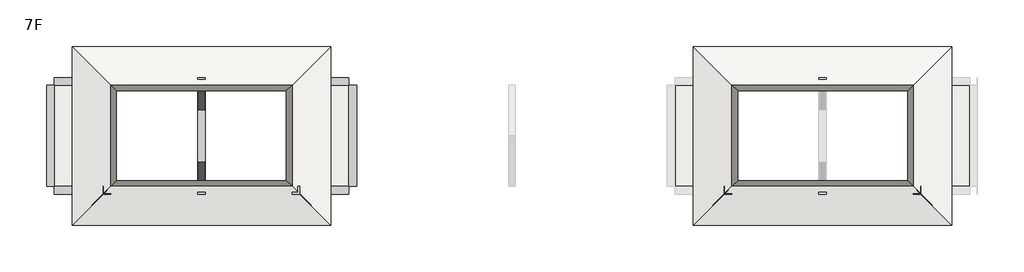
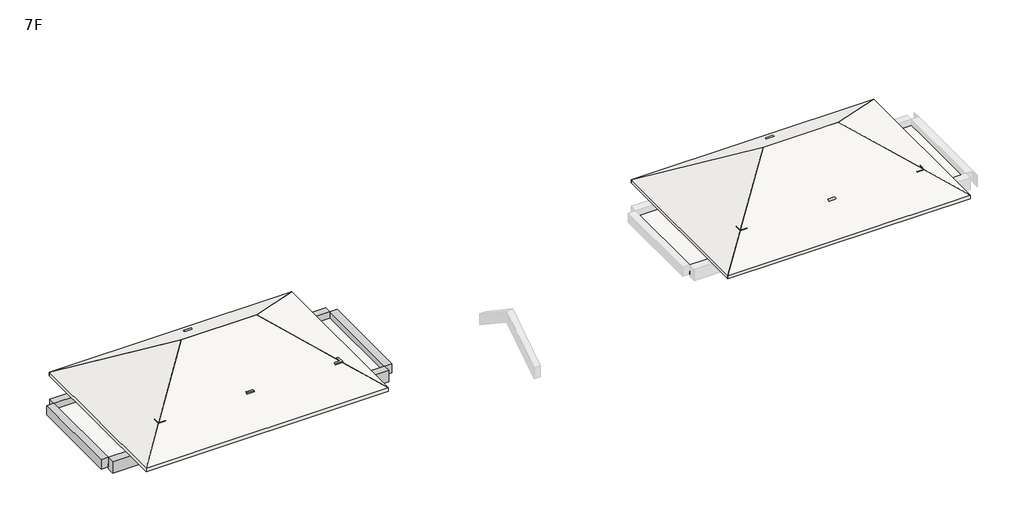
# One storey, part 1 of 2: 15 beams, 9 slabs, 5 columns.
"""IFC4 building model written with IfcOpenShell, lengths in millimetres."""

from ifc_helpers import new_model, si_unit, frame, origin, place, context, project, spatial, polyline, outline, extrude, faceted_brep, element, save

model = new_model("IFC4")

# Units and contexts
model_context = context("Model", 3, world=origin())
ifc_project = project(units=[si_unit("LENGTHUNIT", "METRE", prefix="MILLI")], contexts=[model_context])

# Site, building, storey
site = spatial("IfcSite", under=ifc_project)
building = spatial("IfcBuilding", under=site)
storey = spatial("IfcBuildingStorey", under=building, Name="7F", Elevation=20530.0)

# Beams
placement = place(None, origin())
element("IfcBeam", 1, ObjectType="M_Concrete-Rectangular Beam : 250x400", at=placement, inside=storey, context=model_context, shape_type="SweptSolid", body=[
    extrude(outline(polyline([(9399.8746382, 8450.0000002), (9649.8746382, 8450.0000002), (9649.8746382, 4549.9999996), (9399.8746382, 4549.9999996), (9399.8746382, 8450.0000002)])), frame((0.0, 0.0, 20130.0), z_axis=(0.0, 0.0, 1.0), x_axis=(1.0, 0.0, 0.0)), (0.0, 0.0, 1.0), 400.0),
])
element("IfcBeam", 2, ObjectType="M_Concrete-Rectangular Beam : 250x400", at=placement, inside=storey, context=model_context, shape_type="SweptSolid", body=[
    extrude(outline(polyline([(2050.1253632, 8450.0000002), (2300.1253632, 8450.0000002), (2300.1253632, 4549.9999996), (2050.1253632, 4549.9999996), (2050.1253632, 8450.0000002)])), frame((0.0, 0.0, 20130.0), z_axis=(0.0, 0.0, 1.0), x_axis=(1.0, 0.0, 0.0)), (0.0, 0.0, 1.0), 400.0),
])
element("IfcBeam", 3, ObjectType="M_Concrete-Rectangular Beam : 250x400", at=placement, inside=storey, context=model_context, shape_type="Brep", body=[
    faceted_brep([(5725.0000684, 6499.7375861, 22885.8347272), (5975.0000684, 6499.7375861, 22885.8347272), (5975.0000684, 8449.9999997, 21585.6270796), (5725.0000684, 8449.9999997, 21585.6270796), (5725.0000684, 6277.8536437, 22553.0171854), (5725.0000684, 8449.9999997, 21104.8831887), (5725.0000684, 6499.7375861, 22405.0908362), (5975.0000684, 6277.8536437, 22553.0171854), (5975.0000684, 8449.9999997, 21104.8831887), (5975.0000684, 6499.7375861, 22405.0908362)], [[[0, 1, 2, 3]], [[4, 0, 3, 5, 6]], [[7, 4, 6, 5, 8, 9]], [[1, 7, 9, 8, 2]], [[1, 0, 4, 7]], [[3, 2, 8, 5]]]),
])
element("IfcBeam", 4, ObjectType="M_Concrete-Rectangular Beam : 250x400", at=placement, inside=storey, context=model_context, shape_type="SweptSolid", body=[
    extrude(outline(polyline([(6277.8536437, 22553.0171854), (6499.7375861, 22405.0908362), (4549.9999992, 21105.2330819), (4549.9999992, 21585.9769728), (6499.7375861, 22885.8347272), (6277.8536437, 22553.0171854)])), frame((5725.0000684, 0.0, 0.0), z_axis=(1.0, 0.0, 0.0), x_axis=(0.0, 1.0, 0.0)), (0.0, 0.0, 1.0), 250.0),
])
element("IfcBeam", 5, ObjectType="M_Concrete-Rectangular Beam : 250x400", at=placement, inside=storey, context=model_context, shape_type="Brep", body=[
    faceted_brep([(9629.9825629, 4549.9999992, 21480.0), (9629.9825629, 8724.9999993, 21480.0), (9625.1196449, 8724.9999993, 21480.0), (9508.5592132, 8608.4366337, 21480.0), (9379.9825629, 8608.4366337, 21480.0), (9379.9825629, 8474.9999993, 21480.0), (9379.9825629, 4549.9999992, 21480.0), (9379.9825629, 4549.9999992, 21080.0), (9379.9825629, 8655.7227157, 21448.4751524), (9379.9825629, 8474.9999993, 21448.4751524), (9379.9825629, 8449.9999997, 21448.4751524), (9379.9825629, 8449.9999997, 21080.0), (9629.9825629, 4549.9999992, 21080.0), (9629.9825629, 8449.9999997, 21080.0), (9629.9825629, 8449.9999997, 21448.4751524), (9629.9825629, 8724.9999993, 21448.4751524), (9625.1196449, 8724.9999993, 21448.4751524), (9555.844105, 8655.7227157, 21448.4751524)], [[[0, 1, 2, 3, 4, 5, 6]], [[7, 6, 5, 4, 8, 9, 10, 11]], [[12, 7, 11, 13]], [[1, 0, 12, 13, 14, 15]], [[1, 15, 16, 2]], [[0, 6, 7, 12]], [[10, 14, 13, 11]], [[14, 10, 9, 8, 17, 16, 15]], [[3, 17, 8, 4]], [[17, 3, 2, 16]]]),
])
element("IfcBeam", 6, ObjectType="M_Concrete-Rectangular Beam : 250x400", at=placement, inside=storey, context=model_context, shape_type="SweptSolid", body=[
    extrude(outline(polyline([(21080.0, 2075.0175574), (21080.0, 2325.0175574), (21480.0, 2325.0175574), (21480.0, 2191.5713212), (21402.3014348, 2075.0175574), (21080.0, 2075.0175574)])), frame((0.0, 4549.9999992, 0.0), z_axis=(0.0, 1.0, 0.0), x_axis=(0.0, 0.0, 1.0)), (0.0, 0.0, 1.0), 3887.3000005),
])
element("IfcBeam", 7, ObjectType="M_Concrete-Rectangular Beam : 250x400", at=placement, inside=storey, context=model_context, shape_type="Brep", body=[
    faceted_brep([(5999.9855405, 8474.9999993, 21480.0), (9379.9825629, 8474.9999993, 21480.0), (9379.9825629, 8608.4366337, 21480.0), (5999.9855405, 8608.4366337, 21480.0), (9379.9825629, 8474.9999993, 21448.4751524), (5999.9855405, 8474.9999993, 21080.0), (9349.8746382, 8474.9999993, 21080.0), (9349.8746382, 8474.9999993, 21448.4751524), (9349.8746382, 8724.9999993, 21080.0), (5999.9855405, 8724.9999993, 21080.0), (5999.9855405, 8724.9999993, 21402.2891349), (9349.8746382, 8724.9999993, 21402.2891349), (9379.9825629, 8655.7227157, 21448.4751524), (9349.8746382, 8655.7227157, 21448.4751524)], [[[0, 1, 2, 3]], [[4, 1, 0, 5, 6, 7]], [[8, 6, 5, 9]], [[8, 9, 10, 11]], [[1, 4, 12, 2]], [[7, 6, 8, 11, 13]], [[4, 7, 13, 12]], [[5, 0, 3, 10, 9]], [[3, 2, 12, 13, 11, 10]]]),
    faceted_brep([(2075.0175574, 8474.9999993, 21448.4751524), (2075.0175574, 8474.9999993, 21480.0), (2075.0175574, 8724.7509238, 21480.0), (2075.0175574, 8724.7509238, 21448.4751524), (2350.1253632, 8474.9999993, 21080.0), (2350.1253632, 8474.9999993, 21448.4751524), (2350.1253632, 8655.7227157, 21448.4751524), (2350.1253632, 8724.9999993, 21402.2891349), (2350.1253632, 8724.9999993, 21080.0), (2144.0475031, 8655.7227157, 21448.4751524), (5699.9855405, 8474.9999993, 21480.0), (5699.9855405, 8474.9999993, 21080.0), (5699.9855405, 8724.9999993, 21080.0), (5699.9855405, 8724.9999993, 21402.2891349), (5699.9855405, 8608.4366337, 21480.0), (2191.3347752, 8608.4366337, 21480.0)], [[[0, 1, 2, 3]], [[4, 5, 6, 7, 8]], [[5, 0, 3, 9, 6]], [[10, 11, 12, 13, 14]], [[1, 10, 14, 15, 2]], [[1, 0, 5, 4, 11, 10]], [[4, 8, 12, 11]], [[12, 8, 7, 13]], [[15, 9, 3, 2]], [[9, 15, 14, 13, 7, 6]]]),
])
element("IfcBeam", 8, ObjectType="M_Concrete-Rectangular Beam : 250x400", at=placement, inside=storey, context=model_context, shape_type="SweptSolid", body=[
    extrude(outline(polyline([(4524.9999902, 21080.0), (4274.9999902, 21080.0), (4274.9999902, 21402.6390255), (4391.0385331, 21480.0), (4524.9999902, 21480.0), (4524.9999902, 21080.0)])), frame((5999.9855405, 0.0, 0.0), z_axis=(1.0, 0.0, 0.0), x_axis=(0.0, 1.0, 0.0)), (0.0, 0.0, 1.0), 3349.8890977),
    extrude(outline(polyline([(4524.9999902, 21480.0), (4524.9999902, 21080.0), (4274.9999902, 21080.0), (4274.9999902, 21402.6390255), (4391.0385331, 21480.0), (4524.9999902, 21480.0)])), frame((2350.0175574, 0.0, 0.0), z_axis=(1.0, 0.0, 0.0), x_axis=(0.0, 1.0, 0.0)), (0.0, 0.0, 1.0), 3349.9679831),
])
element("IfcBeam", 9, ObjectType="M_Concrete-Rectangular Beam : 300x400", at=placement, inside=storey, context=model_context, shape_type="SweptSolid", body=[
    extrude(outline(polyline([(165.0, 4549.9999996), (-135.0, 4549.9999996), (-135.0, 8450.0000002), (165.0, 8450.0000002), (165.0, 4549.9999996)])), frame((0.0, 0.0, 20130.0), z_axis=(0.0, 0.0, 1.0), x_axis=(1.0, 0.0, 0.0)), (0.0, 0.0, 1.0), 400.0),
])
element("IfcBeam", 10, ObjectType="M_Concrete-Rectangular Beam : 300x400", at=placement, inside=storey, context=model_context, shape_type="SweptSolid", body=[
    extrude(outline(polyline([(11550.0174941, 8450.0000002), (11850.0174941, 8450.0000002), (11850.0174941, 4549.9999996), (11550.0174941, 4549.9999996), (11550.0174941, 8450.0000002)])), frame((0.0, 0.0, 20130.0), z_axis=(0.0, 0.0, 1.0), x_axis=(1.0, 0.0, 0.0)), (0.0, 0.0, 1.0), 400.0),
])
element("IfcBeam", 11, ObjectType="M_Concrete-Rectangular Beam : 300x400", at=placement, inside=storey, context=model_context, shape_type="Brep", body=[
    faceted_brep([(6000.0, 8450.0000002, 20530.0), (5700.0, 8450.0000002, 20530.0), (5700.0, 4549.9999996, 20530.0), (6000.0, 4550.0000005, 20530.0), (6000.0, 4550.0000005, 20130.0), (6000.0, 8450.0000002, 20130.0), (5700.0, 8450.0000002, 20130.0), (5700.0, 4549.9999996, 20130.0)], [[[0, 1, 2, 3]], [[3, 4, 5, 0]], [[6, 5, 4, 7]], [[1, 6, 7, 2]], [[0, 5, 6, 1]], [[2, 7, 4, 3]]]),
])
element("IfcBeam", 12, ObjectType="M_Concrete-Rectangular Beam : 300x500", at=placement, inside=storey, context=model_context, shape_type="Brep", body=[
    faceted_brep([(164.9649925, 8750.0000002, 20530.0), (164.9649925, 8450.0000002, 20530.0), (2050.1253632, 8450.0000002, 20530.0), (2300.1253632, 8450.0000002, 20530.0), (5700.0000012, 8450.0000002, 20530.0), (5700.0000012, 8750.0000002, 20530.0), (164.9649925, 8450.0000002, 20030.0), (5700.0000012, 8450.0000002, 20030.0), (164.9649925, 8750.0000002, 20030.0), (5700.0000012, 8750.0000002, 20030.0)], [[[0, 1, 2, 3, 4, 5]], [[1, 6, 7, 4, 3, 2]], [[6, 8, 9, 7]], [[8, 0, 5, 9]], [[1, 0, 8, 6]], [[5, 4, 7, 9]]]),
])
element("IfcBeam", 13, ObjectType="M_Concrete-Rectangular Beam : 300x500", at=placement, inside=storey, context=model_context, shape_type="Brep", body=[
    faceted_brep([(164.9649925, 4549.9999996, 20530.0), (164.9649925, 4249.9999996, 20530.0), (5700.0000012, 4249.9999996, 20530.0), (5700.0000012, 4549.9999996, 20530.0), (2300.1253632, 4549.9999996, 20530.0), (2050.1253632, 4549.9999996, 20530.0), (164.9649925, 4249.9999996, 20030.0), (5700.0000012, 4249.9999996, 20030.0), (164.9649925, 4549.9999996, 20030.0), (5700.0000012, 4549.9999996, 20030.0)], [[[0, 1, 2, 3, 4, 5]], [[1, 6, 7, 2]], [[6, 8, 9, 7]], [[8, 0, 5, 4, 3, 9]], [[1, 0, 8, 6]], [[3, 2, 7, 9]]]),
])
element("IfcBeam", 14, ObjectType="M_Concrete-Rectangular Beam : 300x500", at=placement, inside=storey, context=model_context, shape_type="Brep", body=[
    faceted_brep([(6000.0000012, 8750.0000002, 20530.0), (6000.0, 8450.0000002, 20530.0), (9399.8746382, 8450.0000002, 20530.0), (9649.8746382, 8450.0000002, 20530.0), (11550.000003, 8450.0000002, 20530.0), (11550.000003, 8750.0000002, 20530.0), (6000.0000012, 8450.0000002, 20030.0), (11550.000003, 8450.0000002, 20030.0), (6000.0000012, 8750.0000002, 20030.0), (11550.000003, 8750.0000002, 20030.0)], [[[0, 1, 2, 3, 4, 5]], [[1, 6, 7, 4, 3, 2]], [[6, 8, 9, 7]], [[8, 0, 5, 9]], [[8, 6, 1, 0]], [[5, 4, 7, 9]]]),
])
element("IfcBeam", 15, ObjectType="M_Concrete-Rectangular Beam : 300x500", at=placement, inside=storey, context=model_context, shape_type="Brep", body=[
    faceted_brep([(6000.0, 4549.9999996, 20530.0), (6000.0000012, 4249.9999996, 20530.0), (11550.000003, 4249.9999996, 20530.0), (11550.000003, 4549.9999996, 20530.0), (9649.8746382, 4549.9999996, 20530.0), (9399.8746382, 4549.9999996, 20530.0), (6000.0000012, 4249.9999996, 20030.0), (11550.000003, 4249.9999996, 20030.0), (6000.0000012, 4549.9999996, 20030.0), (11550.000003, 4549.9999996, 20030.0)], [[[0, 1, 2, 3, 4, 5]], [[1, 6, 7, 2]], [[6, 8, 9, 7]], [[8, 0, 5, 4, 3, 9]], [[8, 6, 1, 0]], [[3, 2, 7, 9]]]),
])

# Columns
element("IfcColumn", 16, ObjectType="M_Concrete-Rectangular-Column : 300x300", at=placement, inside=storey, context=model_context, shape_type="Brep", body=[
    faceted_brep([(5999.9855405, 4549.9999992, 20530.0), (5999.9855405, 4249.9999992, 20530.0), (5699.9855405, 4249.9999992, 20530.0), (5699.9855405, 4549.9999992, 20530.0), (5699.9855405, 4549.9999992, 21585.9769764), (5999.9855405, 4549.9999992, 21585.9769764), (5999.9855405, 4249.9999992, 21385.9719455), (5999.9855405, 4274.9999902, 21402.6390255), (5999.9855405, 4391.0385331, 21480.0), (5699.9855405, 4391.0385331, 21480.0), (5699.9855405, 4274.9999902, 21402.6390255), (5699.9855405, 4249.9999992, 21385.9719455)], [[[0, 1, 2, 3]], [[0, 3, 4, 5]], [[6, 7, 8, 5, 4, 9, 10, 11]], [[1, 0, 5, 8, 7, 6]], [[2, 1, 6, 11]], [[3, 2, 11, 10, 9, 4]]]),
    faceted_brep([(5999.9855405, 4249.9999992, 21585.9769764), (5999.9855405, 4249.9999992, 21530.1951128), (5999.9855405, 4333.6706899, 21585.9769764), (5699.9855405, 4249.9999992, 21585.9769764), (5699.9855405, 4249.9999992, 21530.1951128), (5699.9855405, 4333.6706899, 21585.9769764)], [[[0, 1, 2]], [[0, 3, 4, 1]], [[4, 3, 5]], [[3, 0, 2, 5]], [[2, 1, 4, 5]]]),
])
element("IfcColumn", 17, ObjectType="M_Concrete-Rectangular-Column : 300x300", at=placement, inside=storey, context=model_context, shape_type="Brep", body=[
    faceted_brep([(5999.9855405, 8749.9999997, 20530.0), (5999.9855405, 8449.9999997, 20530.0), (5699.9855405, 8449.9999997, 20530.0), (5699.9855405, 8749.9999997, 20530.0), (5999.9855405, 8449.9999997, 21585.6270796), (5699.9855405, 8449.9999997, 21585.6270796), (5999.9855405, 8608.4366337, 21480.0), (5999.9855405, 8724.9999993, 21402.2891349), (5999.9855405, 8749.9999997, 21385.6220487), (5699.9855405, 8749.9999997, 21385.6220487), (5699.9855405, 8724.9999993, 21402.2891349), (5699.9855405, 8608.4366337, 21480.0)], [[[0, 1, 2, 3]], [[2, 1, 4, 5]], [[4, 6, 7, 8, 9, 10, 11, 5]], [[1, 0, 8, 7, 6, 4]], [[3, 2, 5, 11, 10, 9]], [[0, 3, 9, 8]]]),
    faceted_brep([(5999.9855405, 8749.9999997, 21529.845216), (5999.9855405, 8749.9999997, 21585.6270796), (5999.9855405, 8666.329309, 21585.6270796), (5699.9855405, 8749.9999997, 21585.6270796), (5699.9855405, 8749.9999997, 21529.845216), (5699.9855405, 8666.329309, 21585.6270796)], [[[0, 1, 2]], [[3, 4, 5]], [[3, 1, 0, 4]], [[1, 3, 5, 2]], [[0, 2, 5, 4]]]),
])
element("IfcColumn", 18, ObjectType="M_Concrete-Rectangular-Column : 300x300", at=placement, inside=storey, context=model_context, shape_type="Brep", body=[
    faceted_brep([(9649.8746382, 4549.9999992, 20530.0), (9649.8746382, 4249.9999992, 20530.0), (9349.8746382, 4249.9999992, 20530.0), (9349.8746382, 4549.9999992, 20530.0), (9649.8746382, 4549.9999992, 21585.6973295), (9649.8746382, 4249.9999992, 21585.6973295), (9649.8746382, 4249.9999992, 21529.9272796), (9649.8746382, 4549.9999992, 21529.9272796), (9649.8746382, 4249.9999992, 21385.7074809), (9649.5941992, 4249.9999992, 21385.8944308), (9649.5941992, 4249.9999992, 21530.1142294), (9349.8746382, 4249.9999992, 21585.6973295), (9349.8746382, 4549.7271047, 21585.6973295), (9349.8746382, 4549.9999992, 21585.6973295), (9566.2153171, 4549.9999992, 21585.6973295), (9566.2153171, 4333.3809801, 21585.6973295), (9649.8746382, 4549.9999992, 21385.7074809)], [[[0, 1, 2, 3]], [[4, 5, 6, 7]], [[2, 1, 8, 9, 10, 6, 5, 11]], [[3, 2, 11, 12, 13]], [[4, 7, 14]], [[5, 4, 14, 15, 12, 11]], [[12, 9, 8, 16, 13]], [[10, 15, 14, 7, 6]], [[9, 12, 15, 10]], [[1, 0, 16, 8]], [[0, 3, 13, 16]]]),
])
element("IfcColumn", 19, ObjectType="M_Concrete-Rectangular-Column : 300x300", at=placement, inside=storey, context=model_context, shape_type="Brep", body=[
    faceted_brep([(2350.1253632, 4549.9999992, 20530.0), (2350.1253632, 4249.9999992, 20530.0), (2050.1253632, 4249.9999992, 20530.0), (2050.1253632, 4549.9999992, 20530.0), (2350.1253632, 4549.9999992, 21544.1224713), (2350.1253632, 4249.9999992, 21544.1224713), (2050.1253632, 4249.9999992, 21544.1224713), (2050.1253632, 4249.9999992, 21529.9272796), (2050.4058022, 4249.9999992, 21530.1142294), (2050.4058022, 4249.9999992, 21385.8944308), (2050.1253632, 4249.9999992, 21385.7074809), (2050.1253632, 4549.9999992, 21544.1224713), (2050.1253632, 4549.9999992, 21529.9272796), (2071.4192316, 4549.9999992, 21544.1224713), (2287.7599104, 4549.9999992, 21544.1224713), (2287.7599104, 4487.360082, 21544.1224713), (2071.4192316, 4271.0139574, 21544.1224713), (2050.1253632, 4549.9999992, 21385.7074809)], [[[0, 1, 2, 3]], [[1, 0, 4, 5]], [[2, 1, 5, 6, 7, 8, 9, 10]], [[6, 11, 12, 7]], [[12, 11, 13]], [[5, 4, 14, 15, 16, 13, 11, 6]], [[9, 15, 14, 17, 10]], [[16, 8, 7, 12, 13]], [[15, 9, 8, 16]], [[3, 2, 10, 17]], [[0, 3, 17, 14, 4]]]),
])
element("IfcColumn", 20, ObjectType="M_Concrete-Rectangular-Column : 300x300", at=placement, inside=storey, context=model_context, shape_type="Brep", body=[
    faceted_brep([(2350.1253632, 8749.9999997, 20530.0), (2350.1253632, 8449.9999997, 20530.0), (2050.1253632, 8449.9999997, 20530.0), (2050.1253632, 8749.9999997, 20530.0), (2350.1253632, 8749.9999997, 21385.6220487), (2350.1253632, 8655.7227157, 21448.4751524), (2350.1253632, 8449.9999997, 21448.4751524), (2050.1253632, 8449.9999997, 21448.4751524), (2050.1253632, 8749.6424915, 21448.4751524), (2050.1253632, 8749.6424915, 21385.8603935), (2050.1253632, 8749.9999997, 21385.6220487), (2144.0475031, 8655.7227157, 21448.4751524)], [[[0, 1, 2, 3]], [[1, 0, 4, 5, 6]], [[2, 1, 6, 7]], [[3, 2, 7, 8, 9, 10]], [[0, 3, 10, 4]], [[7, 6, 5, 11, 8]], [[9, 11, 5, 4, 10]], [[11, 9, 8]]]),
])

# Slabs
element("IfcSlab", 21, ObjectType="120", at=placement, inside=storey, context=model_context, shape_type="Brep", body=[
    faceted_brep([(10849.8264643, 9949.7376449, 20585.7768327), (9555.844105, 8655.7227157, 21448.4751524), (9508.5592132, 8608.4366337, 21480.0), (7400.0000782, 6499.8244256, 22885.7768327), (4300.0000585, 6499.8244256, 22885.7768327), (2191.3347752, 8608.4366337, 21480.0), (2144.0475031, 8655.7227157, 21448.4751524), (2050.1253632, 8749.6424915, 21385.8603935), (850.0000025, 9949.7376449, 20585.7768327), (10849.8264643, 9949.7376449, 20730.0), (850.0000025, 9949.7376449, 20730.0), (4300.0000585, 6499.8244256, 23030.0), (7400.0000782, 6499.8244256, 23030.0)], [[[0, 1, 2, 3, 4, 5, 6, 7, 8]], [[9, 10, 11, 12]], [[0, 8, 10, 9]], [[3, 2, 1, 0, 9, 12]], [[4, 3, 12, 11]], [[8, 7, 6, 5, 4, 11, 10]]]),
])
element("IfcSlab", 22, ObjectType="120", at=placement, inside=storey, context=model_context, shape_type="Brep", body=[
    faceted_brep([(10849.8264639, 9949.7376446, 20585.7802013), (10849.8264639, 3049.7375222, 20585.7802013), (9649.5941992, 4249.9999992, 21385.8944308), (9349.8746382, 4549.7271047, 21585.6973295), (7399.913241, 6499.7375863, 22885.605611), (10849.8264639, 9949.7376446, 20730.0), (7399.913241, 6499.7375863, 23029.8254097), (9566.2153171, 4333.3809801, 21585.6973295), (9649.5941992, 4249.9999992, 21530.1142294), (10849.8264639, 3049.7375222, 20730.0)], [[[0, 1, 2, 3, 4]], [[5, 6, 7, 8, 9]], [[1, 0, 5, 9]], [[4, 3, 2, 1, 9, 8, 7, 6]], [[0, 4, 6, 5]]]),
])
element("IfcSlab", 23, ObjectType="120", at=placement, inside=storey, context=model_context, shape_type="Brep", body=[
    faceted_brep([(10849.8264643, 3049.7375219, 20585.7768327), (850.0000025, 3049.7375219, 20585.7768327), (4300.0000585, 6499.6507412, 22885.7768327), (7400.0000782, 6499.6507412, 22885.7768327), (10849.8264643, 3049.7375219, 20730.0), (7400.0000782, 6499.6507412, 23030.0), (4300.0000585, 6499.6507412, 23030.0), (850.0000025, 3049.7375219, 20730.0)], [[[0, 1, 2, 3]], [[4, 5, 6, 7]], [[1, 0, 4, 7]], [[0, 3, 5, 4]], [[3, 2, 6, 5]], [[2, 1, 7, 6]]]),
])
element("IfcSlab", 24, ObjectType="120", at=placement, inside=storey, context=model_context, shape_type="Brep", body=[
    faceted_brep([(850.1735375, 9949.7376446, 20585.7802013), (4300.0867604, 6499.7375863, 22885.605611), (2287.7599104, 4487.360082, 21544.1224713), (2050.4058022, 4249.9999992, 21385.8944308), (850.1735375, 3049.7375222, 20585.7802013), (850.1735375, 9949.7376446, 20730.0), (850.1735375, 3049.7375222, 20730.0), (2050.4058022, 4249.9999992, 21530.1142294), (2071.4192316, 4271.0139574, 21544.1224713), (4300.0867604, 6499.7375863, 23029.8254097)], [[[0, 1, 2, 3, 4]], [[5, 6, 7, 8, 9]], [[0, 4, 6, 5]], [[4, 3, 2, 1, 9, 8, 7, 6]], [[1, 0, 5, 9]]]),
])
element("IfcSlab", 25, ObjectType="120", at=placement, inside=storey, context=model_context, shape_type="Brep", body=[
    faceted_brep([(34849.8264674, 9949.7376449, 20585.7768327), (33649.8746414, 8749.7556157, 21385.7849755), (33555.8441081, 8655.7227157, 21448.4751524), (33508.5592163, 8608.4366337, 21480.0), (31400.0000814, 6499.8244256, 22885.7768327), (28300.0000617, 6499.8244256, 22885.7768327), (26191.3347784, 8608.4366337, 21480.0), (26144.0475062, 8655.7227157, 21448.4751524), (26050.1253663, 8749.6424915, 21385.8603935), (24850.0000057, 9949.7376449, 20585.7768327), (34849.8264674, 9949.7376449, 20730.0), (24850.0000057, 9949.7376449, 20730.0), (28300.0000617, 6499.8244256, 23030.0), (31400.0000814, 6499.8244256, 23030.0)], [[[0, 1, 2, 3, 4, 5, 6, 7, 8, 9]], [[10, 11, 12, 13]], [[0, 9, 11, 10]], [[4, 3, 2, 1, 0, 10, 13]], [[5, 4, 13, 12]], [[9, 8, 7, 6, 5, 12, 11]]]),
])
element("IfcSlab", 26, ObjectType="120", at=placement, inside=storey, context=model_context, shape_type="Brep", body=[
    faceted_brep([(34849.8264671, 9949.7376446, 20585.7802013), (34849.8264671, 3049.7375222, 20585.7802013), (33649.5942023, 4249.9999992, 21385.8944308), (33412.3407455, 4487.2594281, 21544.0553738), (31399.9132442, 6499.7375863, 22885.605611), (34849.8264671, 9949.7376446, 20730.0), (31399.9132442, 6499.7375863, 23029.8254097), (33628.6814244, 4270.9133035, 21544.0553738), (33649.5942023, 4249.9999992, 21530.1142294), (34849.8264671, 3049.7375222, 20730.0)], [[[0, 1, 2, 3, 4]], [[5, 6, 7, 8, 9]], [[1, 0, 5, 9]], [[4, 3, 2, 1, 9, 8, 7, 6]], [[0, 4, 6, 5]]]),
])
element("IfcSlab", 27, ObjectType="120", at=placement, inside=storey, context=model_context, shape_type="Brep", body=[
    faceted_brep([(34849.8264674, 3049.7375219, 20585.7768327), (24850.0000057, 3049.7375219, 20585.7768327), (28300.0000617, 6499.6507412, 22885.7768327), (31400.0000814, 6499.6507412, 22885.7768327), (34849.8264674, 3049.7375219, 20730.0), (31400.0000814, 6499.6507412, 23030.0), (28300.0000617, 6499.6507412, 23030.0), (24850.0000057, 3049.7375219, 20730.0)], [[[0, 1, 2, 3]], [[4, 5, 6, 7]], [[1, 0, 4, 7]], [[0, 3, 5, 4]], [[3, 2, 6, 5]], [[2, 1, 7, 6]]]),
])
element("IfcSlab", 28, ObjectType="120", at=placement, inside=storey, context=model_context, shape_type="Brep", body=[
    faceted_brep([(24850.1735406, 9949.7376446, 20585.7802013), (28300.0867635, 6499.7375863, 22885.605611), (26287.6592622, 4487.2594281, 21544.0553738), (26050.4058054, 4249.9999992, 21385.8944308), (24850.1735406, 3049.7375222, 20585.7802013), (24850.1735406, 9949.7376446, 20730.0), (24850.1735406, 3049.7375222, 20730.0), (26050.4058054, 4249.9999992, 21530.1142294), (26071.3185833, 4270.9133035, 21544.0553738), (28300.0867635, 6499.7375863, 23029.8254097)], [[[0, 1, 2, 3, 4]], [[5, 6, 7, 8, 9]], [[0, 4, 6, 5]], [[4, 3, 2, 1, 9, 8, 7, 6]], [[1, 0, 5, 9]]]),
])
element("IfcSlab", 29, ObjectType="130", at=placement, inside=storey, context=model_context, shape_type="SweptSolid", body=[
    extrude(outline(polyline([(26050.1253733, 8450.0000002), (26050.1253733, 4549.9999992), (24149.9825174, 4549.9999992), (24149.9825174, 8450.0000002), (26050.1253733, 8450.0000002)])), frame((0.0, 0.0, 20130.0), z_axis=(0.0, 0.0, 1.0), x_axis=(1.0, 0.0, 0.0)), (0.0, 0.0, 1.0), 130.0),
    extrude(outline(polyline([(35535.0000115, 8449.9999997), (35535.0000115, 4549.9999996), (33649.8746418, 4549.9999996), (33649.8746418, 8449.9999997), (35535.0000115, 8449.9999997)])), frame((0.0, 0.0, 20130.0), z_axis=(0.0, 0.0, 1.0), x_axis=(1.0, 0.0, 0.0)), (0.0, 0.0, 1.0), 130.0),
    extrude(outline(polyline([(2050.1253632, 8450.0000002), (2050.1253632, 4549.9999992), (165.0, 4549.9999992), (165.0, 8450.0000002), (2050.1253632, 8450.0000002)])), frame((0.0, 0.0, 20130.0), z_axis=(0.0, 0.0, 1.0), x_axis=(1.0, 0.0, 0.0)), (0.0, 0.0, 1.0), 130.0),
    extrude(outline(polyline([(11550.0174941, 8449.9999997), (11550.0174941, 4549.9999996), (9649.8601776, 4549.9999996), (9649.8601776, 8449.9999997), (11550.0174941, 8449.9999997)])), frame((0.0, 0.0, 20130.0), z_axis=(0.0, 0.0, 1.0), x_axis=(1.0, 0.0, 0.0)), (0.0, 0.0, 1.0), 130.0),
])

save(model, "model.ifc")

# Revit data of these elements
# Type "M_Concrete-Rectangular Beam : 250x400"
#   Length [instance default] = 1524 mm
#   b = 250 mm
#   h = 400 mm
#   Structural Material [instance default] = Concrete, Cast-in-Place gray
#   Assembly Code = ""
# Type "M_Concrete-Rectangular Beam : 300x400"
#   Length [instance default] = 1524 mm
#   b = 300 mm
#   h = 400 mm
#   Structural Material [instance default] = Concrete, Cast-in-Place gray
#   Assembly Code = ""
# Type "M_Concrete-Rectangular Beam : 300x500"
#   Length [instance default] = 1524 mm
#   b = 300 mm
#   h = 500 mm
#   Structural Material [instance default] = Concrete, Cast-in-Place gray
#   Assembly Code = ""
# Type "M_Concrete-Rectangular-Column : 300x300"
#   b = 300 mm
#   h = 300 mm
#   Structural Material [instance default] = Concrete, Cast-in-Place gray
# Type "120"
#   Function = 0
#   Layers, outside or top first: 120 mm "Concrete, Cast-in-Place gray" (function 1)
# Type "130"
#   Function = 0
#   Layers, outside or top first: 130 mm "VM.TM1A-Concrete Wall-M250" (function 1)
# Elements 1, 2 (IfcBeam, "M_Concrete-Rectangular Beam : 250x400")
#   Comments = ""
#   COF_CON__WorkItemNumber = "SH3-A-03F"
#   COF_GEN__Name = "DT2"
#   Structural Material = Concrete, Cast-in-Place gray
#   Phase Created = New Construction
#   Materials on its faces: "Concrete, Cast-in-Place gray"
# Elements 3, 4 (IfcBeam, "M_Concrete-Rectangular Beam : 250x400")
#   Comments = ""
#   COF_CON__WorkItemNumber = "SH3-A-03F"
#   COF_GEN__Name = "DM3"
#   Structural Material = Concrete, Cast-in-Place gray
#   Phase Created = New Construction
#   Materials on its faces: "Concrete, Cast-in-Place gray"
# Elements 5, 6 (IfcBeam, "M_Concrete-Rectangular Beam : 250x400")
#   Comments = ""
#   COF_CON__WorkItemNumber = "SH3-A-03F"
#   COF_GEN__Name = "DM2"
#   Structural Material = Concrete, Cast-in-Place gray
#   Phase Created = New Construction
#   Materials on its faces: "Concrete, Cast-in-Place gray"
# Elements 7, 8 (IfcBeam, "M_Concrete-Rectangular Beam : 250x400")
#   Comments = ""
#   COF_CON__WorkItemNumber = "SH3-A-03F"
#   COF_GEN__Name = "DM1"
#   Structural Material = Concrete, Cast-in-Place gray
#   Phase Created = New Construction
#   Materials on its faces: "Concrete, Cast-in-Place gray"
# Elements 9, 10, 11 (IfcBeam, "M_Concrete-Rectangular Beam : 300x400")
#   Comments = ""
#   COF_CON__WorkItemNumber = "SH3-A-03F"
#   COF_GEN__Name = "DT1"
#   Structural Material = Concrete, Cast-in-Place gray
#   Phase Created = New Construction
#   Materials on its faces: "Concrete, Cast-in-Place gray"
# Elements 12, 13, 14, 15 (IfcBeam, "M_Concrete-Rectangular Beam : 300x500")
#   Comments = ""
#   COF_CON__WorkItemNumber = "SH3-A-03F"
#   COF_GEN__Name = "D2A"
#   Structural Material = Concrete, Cast-in-Place gray
#   Phase Created = New Construction
#   Materials on its faces: "Concrete, Cast-in-Place gray"
# Elements 16, 17 (IfcColumn, "M_Concrete-Rectangular-Column : 300x300")
#   Comments = ""
#   COF_CON__WorkItemNumber = "SH3-A-TF"
#   COF_GEN__Name = "TR4"
#   Structural Material = Concrete, Cast-in-Place gray
#   Phase Created = New Construction
#   Materials on its faces: "Concrete, Cast-in-Place gray"
# Elements 18, 19, 20 (IfcColumn, "M_Concrete-Rectangular-Column : 300x300")
#   Comments = ""
#   COF_CON__WorkItemNumber = "SH3-A-TF"
#   COF_GEN__Name = "TR5"
#   Structural Material = Concrete, Cast-in-Place gray
#   Phase Created = New Construction
#   Materials on its faces: "Concrete, Cast-in-Place gray"
# Elements 21, 23, 25, 27 (IfcSlab, "120")
#   Comments = ""
#   COF_CON__WorkItemNumber = "SH3-A-TF"
#   COF_GEN__Name = "T120"
#   built-in parameter 1001955 = 3.14159 (stored number, unit not read)
#   Height Offset From Level = 200 mm
#   built-in parameter 1001954 = 1
#   Phase Created = New Construction
#   Materials on its faces: "Concrete, Cast-in-Place gray"
# Elements 22, 26 (IfcSlab, "120")
#   Comments = ""
#   COF_CON__WorkItemNumber = "SH3-A-TF"
#   COF_GEN__Name = "T120"
#   built-in parameter 1001955 = 0.785411 (stored number, unit not read)
#   Height Offset From Level = 200 mm
#   built-in parameter 1001954 = 1
#   Phase Created = New Construction
#   Materials on its faces: "Concrete, Cast-in-Place gray"
# Elements 24, 28 (IfcSlab, "120")
#   Comments = ""
#   COF_CON__WorkItemNumber = "SH3-A-TF"
#   COF_GEN__Name = "T120"
#   built-in parameter 1001955 = 2.35618 (stored number, unit not read)
#   Height Offset From Level = 200 mm
#   built-in parameter 1001954 = 1
#   Phase Created = New Construction
#   Materials on its faces: "Concrete, Cast-in-Place gray"
# Element 29 (IfcSlab, "130")
#   COF_GEN__Name = "T130"
#   Height Offset From Level = -270 mm
#   Phase Created = New Construction
#   Materials on its faces: "VM.TM1A-Concrete Wall-M250"
# Materials
#   "Concrete, Cast-in-Place gray": class "Concrete", colour RGB 207 208 204, transparency 0, Description = "Cast-in-place concrete", Cost = 0
#   "VM.TM1A-Concrete Wall-M250": class "Concrete", colour RGB 192 192 192, transparency 0, Description = "Cast-in-place concrete", Cost = 0
